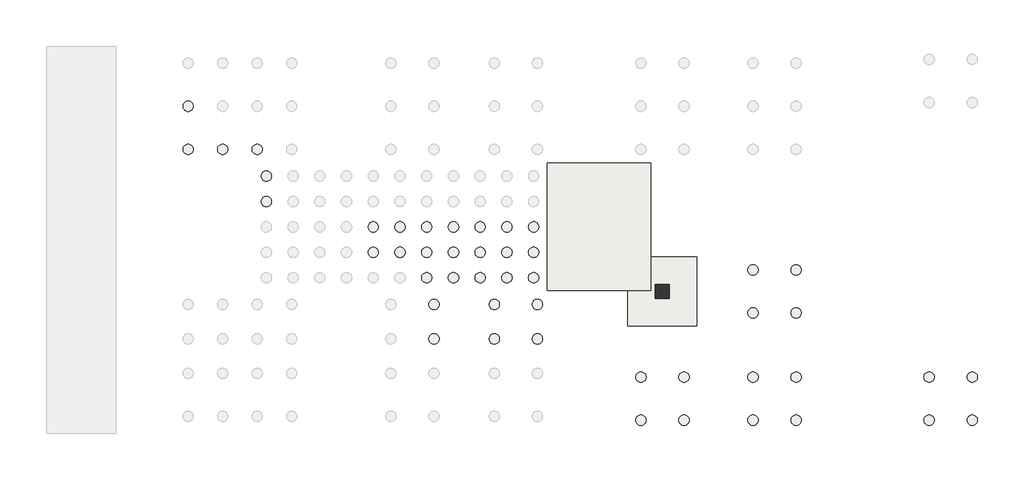
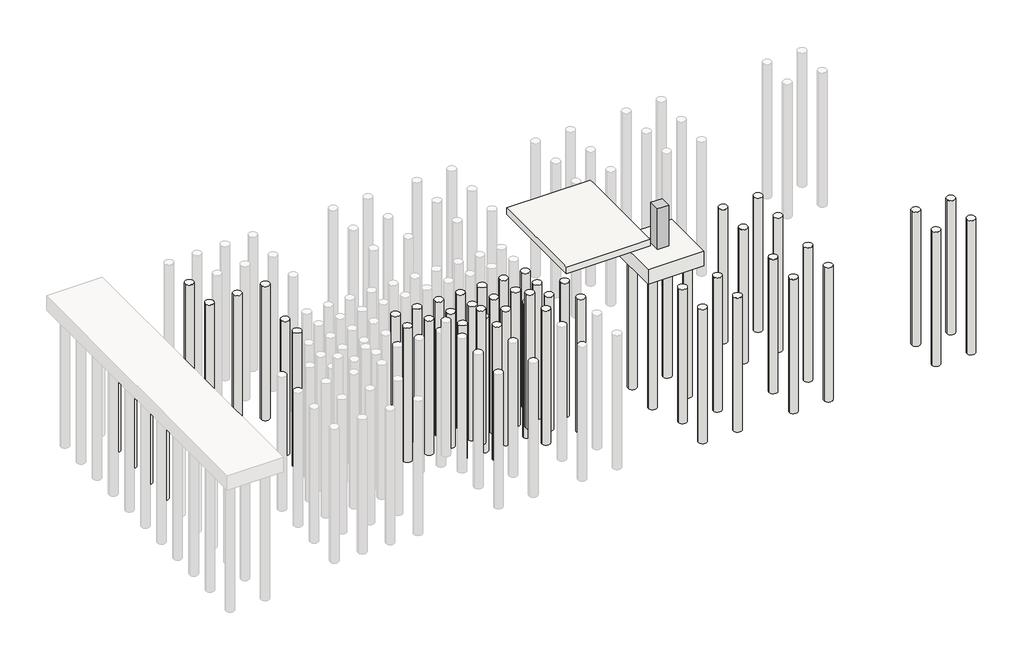
# One storey, part 2 of 3: 57 slabs, 1 column.
"""IFC4 building model written with IfcOpenShell, lengths in millimetres."""

from ifc_helpers import new_model, si_unit, point, frame, frame_2d, origin, place, context, project, spatial, polyline, circle_curve, trimmed, segment, composite_curve, outline, extrude, faceted_brep, element, save

model = new_model("IFC4")

# Units and contexts
model_context = context("Model", 3, world=origin())
ifc_project = project(units=[si_unit("LENGTHUNIT", "METRE", prefix="MILLI")], contexts=[model_context])

# Site, building, storey
site = spatial("IfcSite", under=ifc_project)
building = spatial("IfcBuilding", under=site)
storey = spatial("IfcBuildingStorey", under=building, Name="B.O.F(FDN)", Elevation=-2500.0279945)

# Column
placement = place(None, origin())
element("IfcColumn", 1, ObjectType="RC_Pedestal : H_SC_ACC_PED_W800xL800", at=placement, inside=storey, context=model_context, shape_type="SweptSolid", body=[
    extrude(outline(polyline([(33894.0, 26599.5208589), (33094.0, 26599.5208589), (33094.0, 27399.5208589), (33894.0, 27399.5208589), (33894.0, 26599.5208589)])), frame((0.0, 0.0, -2500.0279945), z_axis=(0.0, 0.0, 1.0), x_axis=(1.0, 0.0, 0.0)), (0.0, 0.0, 1.0), 3100.0),
])

# Slabs
element("IfcSlab", 2, ObjectType="H_SF_ACP_Pit Slab T500", at=placement, inside=storey, context=model_context, shape_type="Brep", body=[
    faceted_brep([(26830.0, 34449.5208589, -2400.0279945), (32830.0, 34449.5208589, -2400.0279945), (32830.0, 27049.5208589, -2400.0279945), (26830.0, 27049.5208589, -2400.0279945), (26830.0, 34449.5208589, -1900.0279945), (26830.0, 34059.5208589, -1900.0279945), (26830.0, 27439.5208589, -1900.0279945), (26830.0, 27049.5208589, -1900.0279945), (32830.0, 27049.5208589, -1900.0279945), (32830.0, 27439.5208589, -1900.0279945), (32830.0, 34059.5208589, -1900.0279945), (32830.0, 34449.5208589, -1900.0279945)], [[[0, 1, 2, 3]], [[4, 5, 6, 7, 8, 9, 10, 11]], [[1, 0, 4, 11]], [[2, 1, 11, 10, 9, 8]], [[3, 2, 8, 7]], [[0, 3, 7, 6, 5, 4]]]),
])
element("IfcSlab", 3, ObjectType="Foundation Rectangular(Non-Pile) : H_SF_ACF_W4000xL4000xT1100_Protection", at=placement, inside=storey, context=model_context, shape_type="SweptSolid", body=[
    extrude(outline(polyline([(35500.0, 28999.5208589), (35500.0, 24999.5208589), (31500.0, 24999.5208589), (31500.0, 28999.5208589), (35500.0, 28999.5208589)])), frame((0.0, 0.0, -3600.0279945), z_axis=(0.0, 0.0, 1.0), x_axis=(1.0, 0.0, 0.0)), (0.0, 0.0, 1.0), 1100.0),
])
element("IfcSlab", 4, ObjectType="Pile : H_SF_API_Steel Pile D508x12t_L10m", at=placement, inside=storey, context=model_context, shape_type="SweptSolid", body=[
    extrude(outline(composite_curve([segment(trimmed(circle_curve(frame_2d((1035.0, 38249.5208589)), 300.0), [point((1335.0, 38249.5208589))], [point((735.0, 38249.5208589))], False, "CARTESIAN"), True, "CONTINUOUS"), segment(trimmed(circle_curve(frame_2d((1035.0, 38249.5208589)), 300.0), [point((735.0, 38249.5208589))], [point((1335.0, 38249.5208589))], False, "CARTESIAN"), True, "CONTINUOUS")], self_intersect=False)), frame((0.0, 0.0, -13500.0279945), z_axis=(0.0, 0.0, 1.0), x_axis=(1.0, 0.0, 0.0)), (0.0, 0.0, 1.0), 10150.0),
])
element("IfcSlab", 5, ObjectType="Pile : H_SF_API_Steel Pile D508x12t_L10m", at=placement, inside=storey, context=model_context, shape_type="SweptSolid", body=[
    extrude(outline(composite_curve([segment(trimmed(circle_curve(frame_2d((1035.0, 36249.5208589)), 300.0), [point((1335.0, 36249.5208589))], [point((735.0, 36249.5208589))], False, "CARTESIAN"), True, "CONTINUOUS"), segment(trimmed(circle_curve(frame_2d((1035.0, 36249.5208589)), 300.0), [point((735.0, 36249.5208589))], [point((1335.0, 36249.5208589))], False, "CARTESIAN"), True, "CONTINUOUS")], self_intersect=False)), frame((0.0, 0.0, -13500.0279945), z_axis=(0.0, 0.0, 1.0), x_axis=(1.0, 0.0, 0.0)), (0.0, 0.0, 1.0), 10150.0),
])
element("IfcSlab", 6, ObjectType="Pile : H_SF_API_Steel Pile D508x12t_L10m", at=placement, inside=storey, context=model_context, shape_type="SweptSolid", body=[
    extrude(outline(composite_curve([segment(trimmed(circle_curve(frame_2d((1035.0, 34249.5208589)), 300.0), [point((1335.0, 34249.5208589))], [point((735.0, 34249.5208589))], False, "CARTESIAN"), True, "CONTINUOUS"), segment(trimmed(circle_curve(frame_2d((1035.0, 34249.5208589)), 300.0), [point((735.0, 34249.5208589))], [point((1335.0, 34249.5208589))], False, "CARTESIAN"), True, "CONTINUOUS")], self_intersect=False)), frame((0.0, 0.0, -13500.0279945), z_axis=(0.0, 0.0, 1.0), x_axis=(1.0, 0.0, 0.0)), (0.0, 0.0, 1.0), 10150.0),
])
element("IfcSlab", 7, ObjectType="Pile : H_SF_API_Steel Pile D508x12t_L10m", at=placement, inside=storey, context=model_context, shape_type="SweptSolid", body=[
    extrude(outline(composite_curve([segment(trimmed(circle_curve(frame_2d((1035.0, 32249.5208589)), 300.0), [point((1335.0, 32249.5208589))], [point((735.0, 32249.5208589))], False, "CARTESIAN"), True, "CONTINUOUS"), segment(trimmed(circle_curve(frame_2d((1035.0, 32249.5208589)), 300.0), [point((735.0, 32249.5208589))], [point((1335.0, 32249.5208589))], False, "CARTESIAN"), True, "CONTINUOUS")], self_intersect=False)), frame((0.0, 0.0, -13500.0279945), z_axis=(0.0, 0.0, 1.0), x_axis=(1.0, 0.0, 0.0)), (0.0, 0.0, 1.0), 10150.0),
])
element("IfcSlab", 8, ObjectType="Pile : H_SF_API_Steel Pile D508x12t_L10m", at=placement, inside=storey, context=model_context, shape_type="SweptSolid", body=[
    extrude(outline(composite_curve([segment(trimmed(circle_curve(frame_2d((20250.0, 24249.5208589)), 300.0), [point((20550.0, 24249.5208589))], [point((19950.0, 24249.5208589))], False, "CARTESIAN"), True, "CONTINUOUS"), segment(trimmed(circle_curve(frame_2d((20250.0, 24249.5208589)), 300.0), [point((19950.0, 24249.5208589))], [point((20550.0, 24249.5208589))], False, "CARTESIAN"), True, "CONTINUOUS")], self_intersect=False)), frame((0.0, 0.0, -12400.0279945), z_axis=(0.0, 0.0, 1.0), x_axis=(1.0, 0.0, 0.0)), (0.0, 0.0, 1.0), 10150.0),
])
element("IfcSlab", 9, ObjectType="Pile : H_SF_API_Steel Pile D508x12t_L10m", at=placement, inside=storey, context=model_context, shape_type="SweptSolid", body=[
    extrude(outline(composite_curve([segment(trimmed(circle_curve(frame_2d((20250.0, 26249.5208589)), 300.0), [point((20550.0, 26249.5208589))], [point((19950.0, 26249.5208589))], False, "CARTESIAN"), True, "CONTINUOUS"), segment(trimmed(circle_curve(frame_2d((20250.0, 26249.5208589)), 300.0), [point((19950.0, 26249.5208589))], [point((20550.0, 26249.5208589))], False, "CARTESIAN"), True, "CONTINUOUS")], self_intersect=False)), frame((0.0, 0.0, -12400.0279945), z_axis=(0.0, 0.0, 1.0), x_axis=(1.0, 0.0, 0.0)), (0.0, 0.0, 1.0), 10150.0),
])
element("IfcSlab", 10, ObjectType="Pile : H_SF_API_Steel Pile D508x12t_L10m", at=placement, inside=storey, context=model_context, shape_type="SweptSolid", body=[
    extrude(outline(composite_curve([segment(trimmed(circle_curve(frame_2d((23750.0, 24249.5208589)), 300.0), [point((23450.0, 24249.5208589))], [point((24050.0, 24249.5208589))], False, "CARTESIAN"), True, "CONTINUOUS"), segment(trimmed(circle_curve(frame_2d((23750.0, 24249.5208589)), 300.0), [point((24050.0, 24249.5208589))], [point((23450.0, 24249.5208589))], False, "CARTESIAN"), True, "CONTINUOUS")], self_intersect=False)), frame((0.0, 0.0, -12400.0279945), z_axis=(0.0, 0.0, 1.0), x_axis=(1.0, 0.0, 0.0)), (0.0, 0.0, 1.0), 10150.0),
])
element("IfcSlab", 11, ObjectType="Pile : H_SF_API_Steel Pile D508x12t_L10m", at=placement, inside=storey, context=model_context, shape_type="SweptSolid", body=[
    extrude(outline(composite_curve([segment(trimmed(circle_curve(frame_2d((26250.0, 26249.5208589)), 300.0), [point((26550.0, 26249.5208589))], [point((25950.0, 26249.5208589))], False, "CARTESIAN"), True, "CONTINUOUS"), segment(trimmed(circle_curve(frame_2d((26250.0, 26249.5208589)), 300.0), [point((25950.0, 26249.5208589))], [point((26550.0, 26249.5208589))], False, "CARTESIAN"), True, "CONTINUOUS")], self_intersect=False)), frame((0.0, 0.0, -12400.0279945), z_axis=(0.0, 0.0, 1.0), x_axis=(1.0, 0.0, 0.0)), (0.0, 0.0, 1.0), 10150.0),
])
element("IfcSlab", 12, ObjectType="Pile : H_SF_API_Steel Pile D508x12t_L10m", at=placement, inside=storey, context=model_context, shape_type="SweptSolid", body=[
    extrude(outline(composite_curve([segment(trimmed(circle_curve(frame_2d((23750.0, 26249.5208589)), 300.0), [point((23450.0, 26249.5208589))], [point((24050.0, 26249.5208589))], False, "CARTESIAN"), True, "CONTINUOUS"), segment(trimmed(circle_curve(frame_2d((23750.0, 26249.5208589)), 300.0), [point((24050.0, 26249.5208589))], [point((23450.0, 26249.5208589))], False, "CARTESIAN"), True, "CONTINUOUS")], self_intersect=False)), frame((0.0, 0.0, -12400.0279945), z_axis=(0.0, 0.0, 1.0), x_axis=(1.0, 0.0, 0.0)), (0.0, 0.0, 1.0), 10150.0),
])
element("IfcSlab", 13, ObjectType="Pile : H_SF_API_Steel Pile D508x12t_L10m", at=placement, inside=storey, context=model_context, shape_type="SweptSolid", body=[
    extrude(outline(composite_curve([segment(trimmed(circle_curve(frame_2d((34750.0, 19529.5208589)), 300.0), [point((35050.0, 19529.5208589))], [point((34450.0, 19529.5208589))], False, "CARTESIAN"), True, "CONTINUOUS"), segment(trimmed(circle_curve(frame_2d((34750.0, 19529.5208589)), 300.0), [point((34450.0, 19529.5208589))], [point((35050.0, 19529.5208589))], False, "CARTESIAN"), True, "CONTINUOUS")], self_intersect=False)), frame((0.0, 0.0, -12400.0279945), z_axis=(0.0, 0.0, 1.0), x_axis=(1.0, 0.0, 0.0)), (0.0, 0.0, 1.0), 10150.0),
])
element("IfcSlab", 14, ObjectType="Pile : H_SF_API_Steel Pile D508x12t_L10m", at=placement, inside=storey, context=model_context, shape_type="SweptSolid", body=[
    extrude(outline(composite_curve([segment(trimmed(circle_curve(frame_2d((32250.0, 19529.5208589)), 300.0), [point((31950.0, 19529.5208589))], [point((32550.0, 19529.5208589))], False, "CARTESIAN"), True, "CONTINUOUS"), segment(trimmed(circle_curve(frame_2d((32250.0, 19529.5208589)), 300.0), [point((32550.0, 19529.5208589))], [point((31950.0, 19529.5208589))], False, "CARTESIAN"), True, "CONTINUOUS")], self_intersect=False)), frame((0.0, 0.0, -12400.0279945), z_axis=(0.0, 0.0, 1.0), x_axis=(1.0, 0.0, 0.0)), (0.0, 0.0, 1.0), 10150.0),
])
element("IfcSlab", 15, ObjectType="Pile : H_SF_API_Steel Pile D508x12t_L10m", at=placement, inside=storey, context=model_context, shape_type="SweptSolid", body=[
    extrude(outline(composite_curve([segment(trimmed(circle_curve(frame_2d((34750.0, 22029.5208589)), 300.0), [point((35050.0, 22029.5208589))], [point((34450.0, 22029.5208589))], False, "CARTESIAN"), True, "CONTINUOUS"), segment(trimmed(circle_curve(frame_2d((34750.0, 22029.5208589)), 300.0), [point((34450.0, 22029.5208589))], [point((35050.0, 22029.5208589))], False, "CARTESIAN"), True, "CONTINUOUS")], self_intersect=False)), frame((0.0, 0.0, -12400.0279945), z_axis=(0.0, 0.0, 1.0), x_axis=(1.0, 0.0, 0.0)), (0.0, 0.0, 1.0), 10150.0),
])
element("IfcSlab", 16, ObjectType="Pile : H_SF_API_Steel Pile D508x12t_L10m", at=placement, inside=storey, context=model_context, shape_type="SweptSolid", body=[
    extrude(outline(composite_curve([segment(trimmed(circle_curve(frame_2d((32250.0, 22029.5208589)), 300.0), [point((31950.0, 22029.5208589))], [point((32550.0, 22029.5208589))], False, "CARTESIAN"), True, "CONTINUOUS"), segment(trimmed(circle_curve(frame_2d((32250.0, 22029.5208589)), 300.0), [point((32550.0, 22029.5208589))], [point((31950.0, 22029.5208589))], False, "CARTESIAN"), True, "CONTINUOUS")], self_intersect=False)), frame((0.0, 0.0, -12400.0279945), z_axis=(0.0, 0.0, 1.0), x_axis=(1.0, 0.0, 0.0)), (0.0, 0.0, 1.0), 10150.0),
])
element("IfcSlab", 17, ObjectType="Pile : H_SF_API_Steel Pile D508x12t_L10m", at=placement, inside=storey, context=model_context, shape_type="SweptSolid", body=[
    extrude(outline(composite_curve([segment(trimmed(circle_curve(frame_2d((34750.0, 25749.5208589)), 300.0), [point((35050.0, 25749.5208589))], [point((34450.0, 25749.5208589))], False, "CARTESIAN"), True, "CONTINUOUS"), segment(trimmed(circle_curve(frame_2d((34750.0, 25749.5208589)), 300.0), [point((34450.0, 25749.5208589))], [point((35050.0, 25749.5208589))], False, "CARTESIAN"), True, "CONTINUOUS")], self_intersect=False)), frame((0.0, 0.0, -13600.0279945), z_axis=(0.0, 0.0, 1.0), x_axis=(1.0, 0.0, 0.0)), (0.0, 0.0, 1.0), 10150.0),
])
element("IfcSlab", 18, ObjectType="Pile : H_SF_API_Steel Pile D508x12t_L10m", at=placement, inside=storey, context=model_context, shape_type="SweptSolid", body=[
    extrude(outline(composite_curve([segment(trimmed(circle_curve(frame_2d((32250.0, 25749.5208589)), 300.0), [point((31950.0, 25749.5208589))], [point((32550.0, 25749.5208589))], False, "CARTESIAN"), True, "CONTINUOUS"), segment(trimmed(circle_curve(frame_2d((32250.0, 25749.5208589)), 300.0), [point((32550.0, 25749.5208589))], [point((31950.0, 25749.5208589))], False, "CARTESIAN"), True, "CONTINUOUS")], self_intersect=False)), frame((0.0, 0.0, -13600.0279945), z_axis=(0.0, 0.0, 1.0), x_axis=(1.0, 0.0, 0.0)), (0.0, 0.0, 1.0), 10150.0),
])
element("IfcSlab", 19, ObjectType="Pile : H_SF_API_Steel Pile D508x12t_L10m", at=placement, inside=storey, context=model_context, shape_type="SweptSolid", body=[
    extrude(outline(composite_curve([segment(trimmed(circle_curve(frame_2d((34750.0, 28249.5208589)), 300.0), [point((35050.0, 28249.5208589))], [point((34450.0, 28249.5208589))], False, "CARTESIAN"), True, "CONTINUOUS"), segment(trimmed(circle_curve(frame_2d((34750.0, 28249.5208589)), 300.0), [point((34450.0, 28249.5208589))], [point((35050.0, 28249.5208589))], False, "CARTESIAN"), True, "CONTINUOUS")], self_intersect=False)), frame((0.0, 0.0, -13600.0279945), z_axis=(0.0, 0.0, 1.0), x_axis=(1.0, 0.0, 0.0)), (0.0, 0.0, 1.0), 10150.0),
])
element("IfcSlab", 20, ObjectType="Pile : H_SF_API_Steel Pile D508x12t_L10m", at=placement, inside=storey, context=model_context, shape_type="SweptSolid", body=[
    extrude(outline(composite_curve([segment(trimmed(circle_curve(frame_2d((32250.0, 28249.5208589)), 300.0), [point((31950.0, 28249.5208589))], [point((32550.0, 28249.5208589))], False, "CARTESIAN"), True, "CONTINUOUS"), segment(trimmed(circle_curve(frame_2d((32250.0, 28249.5208589)), 300.0), [point((32550.0, 28249.5208589))], [point((31950.0, 28249.5208589))], False, "CARTESIAN"), True, "CONTINUOUS")], self_intersect=False)), frame((0.0, 0.0, -13600.0279945), z_axis=(0.0, 0.0, 1.0), x_axis=(1.0, 0.0, 0.0)), (0.0, 0.0, 1.0), 10150.0),
])
element("IfcSlab", 21, ObjectType="Pile : H_SF_API_Steel Pile D508x12t_L10m", at=placement, inside=storey, context=model_context, shape_type="SweptSolid", body=[
    extrude(outline(composite_curve([segment(trimmed(circle_curve(frame_2d((41250.0, 25749.5208589)), 300.0), [point((41550.0, 25749.5208589))], [point((40950.0, 25749.5208589))], False, "CARTESIAN"), True, "CONTINUOUS"), segment(trimmed(circle_curve(frame_2d((41250.0, 25749.5208589)), 300.0), [point((40950.0, 25749.5208589))], [point((41550.0, 25749.5208589))], False, "CARTESIAN"), True, "CONTINUOUS")], self_intersect=False)), frame((0.0, 0.0, -12400.0279945), z_axis=(0.0, 0.0, 1.0), x_axis=(1.0, 0.0, 0.0)), (0.0, 0.0, 1.0), 10150.0),
])
element("IfcSlab", 22, ObjectType="Pile : H_SF_API_Steel Pile D508x12t_L10m", at=placement, inside=storey, context=model_context, shape_type="SweptSolid", body=[
    extrude(outline(composite_curve([segment(trimmed(circle_curve(frame_2d((38750.0, 25749.5208589)), 300.0), [point((38450.0, 25749.5208589))], [point((39050.0, 25749.5208589))], False, "CARTESIAN"), True, "CONTINUOUS"), segment(trimmed(circle_curve(frame_2d((38750.0, 25749.5208589)), 300.0), [point((39050.0, 25749.5208589))], [point((38450.0, 25749.5208589))], False, "CARTESIAN"), True, "CONTINUOUS")], self_intersect=False)), frame((0.0, 0.0, -12400.0279945), z_axis=(0.0, 0.0, 1.0), x_axis=(1.0, 0.0, 0.0)), (0.0, 0.0, 1.0), 10150.0),
])
element("IfcSlab", 23, ObjectType="Pile : H_SF_API_Steel Pile D508x12t_L10m", at=placement, inside=storey, context=model_context, shape_type="SweptSolid", body=[
    extrude(outline(composite_curve([segment(trimmed(circle_curve(frame_2d((41250.0, 28249.5208589)), 300.0), [point((41550.0, 28249.5208589))], [point((40950.0, 28249.5208589))], False, "CARTESIAN"), True, "CONTINUOUS"), segment(trimmed(circle_curve(frame_2d((41250.0, 28249.5208589)), 300.0), [point((40950.0, 28249.5208589))], [point((41550.0, 28249.5208589))], False, "CARTESIAN"), True, "CONTINUOUS")], self_intersect=False)), frame((0.0, 0.0, -12400.0279945), z_axis=(0.0, 0.0, 1.0), x_axis=(1.0, 0.0, 0.0)), (0.0, 0.0, 1.0), 10150.0),
])
element("IfcSlab", 24, ObjectType="Pile : H_SF_API_Steel Pile D508x12t_L10m", at=placement, inside=storey, context=model_context, shape_type="SweptSolid", body=[
    extrude(outline(composite_curve([segment(trimmed(circle_curve(frame_2d((38750.0, 28249.5208589)), 300.0), [point((38450.0, 28249.5208589))], [point((39050.0, 28249.5208589))], False, "CARTESIAN"), True, "CONTINUOUS"), segment(trimmed(circle_curve(frame_2d((38750.0, 28249.5208589)), 300.0), [point((39050.0, 28249.5208589))], [point((38450.0, 28249.5208589))], False, "CARTESIAN"), True, "CONTINUOUS")], self_intersect=False)), frame((0.0, 0.0, -12400.0279945), z_axis=(0.0, 0.0, 1.0), x_axis=(1.0, 0.0, 0.0)), (0.0, 0.0, 1.0), 10150.0),
])
element("IfcSlab", 25, ObjectType="Pile : H_SF_API_Steel Pile D508x12t_L10m", at=placement, inside=storey, context=model_context, shape_type="SweptSolid", body=[
    extrude(outline(composite_curve([segment(trimmed(circle_curve(frame_2d((41250.0, 19529.5208589)), 300.0), [point((41550.0, 19529.5208589))], [point((40950.0, 19529.5208589))], False, "CARTESIAN"), True, "CONTINUOUS"), segment(trimmed(circle_curve(frame_2d((41250.0, 19529.5208589)), 300.0), [point((40950.0, 19529.5208589))], [point((41550.0, 19529.5208589))], False, "CARTESIAN"), True, "CONTINUOUS")], self_intersect=False)), frame((0.0, 0.0, -12400.0279945), z_axis=(0.0, 0.0, 1.0), x_axis=(1.0, 0.0, 0.0)), (0.0, 0.0, 1.0), 10150.0),
])
element("IfcSlab", 26, ObjectType="Pile : H_SF_API_Steel Pile D508x12t_L10m", at=placement, inside=storey, context=model_context, shape_type="SweptSolid", body=[
    extrude(outline(composite_curve([segment(trimmed(circle_curve(frame_2d((38750.0, 19529.5208589)), 300.0), [point((38450.0, 19529.5208589))], [point((39050.0, 19529.5208589))], False, "CARTESIAN"), True, "CONTINUOUS"), segment(trimmed(circle_curve(frame_2d((38750.0, 19529.5208589)), 300.0), [point((39050.0, 19529.5208589))], [point((38450.0, 19529.5208589))], False, "CARTESIAN"), True, "CONTINUOUS")], self_intersect=False)), frame((0.0, 0.0, -12400.0279945), z_axis=(0.0, 0.0, 1.0), x_axis=(1.0, 0.0, 0.0)), (0.0, 0.0, 1.0), 10150.0),
])
element("IfcSlab", 27, ObjectType="Pile : H_SF_API_Steel Pile D508x12t_L10m", at=placement, inside=storey, context=model_context, shape_type="SweptSolid", body=[
    extrude(outline(composite_curve([segment(trimmed(circle_curve(frame_2d((41250.0, 22029.5208589)), 300.0), [point((41550.0, 22029.5208589))], [point((40950.0, 22029.5208589))], False, "CARTESIAN"), True, "CONTINUOUS"), segment(trimmed(circle_curve(frame_2d((41250.0, 22029.5208589)), 300.0), [point((40950.0, 22029.5208589))], [point((41550.0, 22029.5208589))], False, "CARTESIAN"), True, "CONTINUOUS")], self_intersect=False)), frame((0.0, 0.0, -12400.0279945), z_axis=(0.0, 0.0, 1.0), x_axis=(1.0, 0.0, 0.0)), (0.0, 0.0, 1.0), 10150.0),
])
element("IfcSlab", 28, ObjectType="Pile : H_SF_API_Steel Pile D508x12t_L10m", at=placement, inside=storey, context=model_context, shape_type="SweptSolid", body=[
    extrude(outline(composite_curve([segment(trimmed(circle_curve(frame_2d((38750.0, 22029.5208589)), 300.0), [point((38450.0, 22029.5208589))], [point((39050.0, 22029.5208589))], False, "CARTESIAN"), True, "CONTINUOUS"), segment(trimmed(circle_curve(frame_2d((38750.0, 22029.5208589)), 300.0), [point((39050.0, 22029.5208589))], [point((38450.0, 22029.5208589))], False, "CARTESIAN"), True, "CONTINUOUS")], self_intersect=False)), frame((0.0, 0.0, -12400.0279945), z_axis=(0.0, 0.0, 1.0), x_axis=(1.0, 0.0, 0.0)), (0.0, 0.0, 1.0), 10150.0),
])
element("IfcSlab", 29, ObjectType="Pile : H_SF_API_Steel Pile D508x12t_L10m", at=placement, inside=storey, context=model_context, shape_type="SweptSolid", body=[
    extrude(outline(composite_curve([segment(trimmed(circle_curve(frame_2d((51465.0, 19529.5208589)), 300.0), [point((51765.0, 19529.5208589))], [point((51165.0, 19529.5208589))], False, "CARTESIAN"), True, "CONTINUOUS"), segment(trimmed(circle_curve(frame_2d((51465.0, 19529.5208589)), 300.0), [point((51165.0, 19529.5208589))], [point((51765.0, 19529.5208589))], False, "CARTESIAN"), True, "CONTINUOUS")], self_intersect=False)), frame((0.0, 0.0, -12400.0279945), z_axis=(0.0, 0.0, 1.0), x_axis=(1.0, 0.0, 0.0)), (0.0, 0.0, 1.0), 10150.0),
])
element("IfcSlab", 30, ObjectType="Pile : H_SF_API_Steel Pile D508x12t_L10m", at=placement, inside=storey, context=model_context, shape_type="SweptSolid", body=[
    extrude(outline(composite_curve([segment(trimmed(circle_curve(frame_2d((48965.0, 19529.5208589)), 300.0), [point((48665.0, 19529.5208589))], [point((49265.0, 19529.5208589))], False, "CARTESIAN"), True, "CONTINUOUS"), segment(trimmed(circle_curve(frame_2d((48965.0, 19529.5208589)), 300.0), [point((49265.0, 19529.5208589))], [point((48665.0, 19529.5208589))], False, "CARTESIAN"), True, "CONTINUOUS")], self_intersect=False)), frame((0.0, 0.0, -12400.0279945), z_axis=(0.0, 0.0, 1.0), x_axis=(1.0, 0.0, 0.0)), (0.0, 0.0, 1.0), 10150.0),
])
element("IfcSlab", 31, ObjectType="Pile : H_SF_API_Steel Pile D508x12t_L10m", at=placement, inside=storey, context=model_context, shape_type="SweptSolid", body=[
    extrude(outline(composite_curve([segment(trimmed(circle_curve(frame_2d((51465.0, 22029.5208589)), 300.0), [point((51765.0, 22029.5208589))], [point((51165.0, 22029.5208589))], False, "CARTESIAN"), True, "CONTINUOUS"), segment(trimmed(circle_curve(frame_2d((51465.0, 22029.5208589)), 300.0), [point((51165.0, 22029.5208589))], [point((51765.0, 22029.5208589))], False, "CARTESIAN"), True, "CONTINUOUS")], self_intersect=False)), frame((0.0, 0.0, -12400.0279945), z_axis=(0.0, 0.0, 1.0), x_axis=(1.0, 0.0, 0.0)), (0.0, 0.0, 1.0), 10150.0),
])
element("IfcSlab", 32, ObjectType="Pile : H_SF_API_Steel Pile D508x12t_L10m", at=placement, inside=storey, context=model_context, shape_type="SweptSolid", body=[
    extrude(outline(composite_curve([segment(trimmed(circle_curve(frame_2d((48965.0, 22029.5208589)), 300.0), [point((48665.0, 22029.5208589))], [point((49265.0, 22029.5208589))], False, "CARTESIAN"), True, "CONTINUOUS"), segment(trimmed(circle_curve(frame_2d((48965.0, 22029.5208589)), 300.0), [point((49265.0, 22029.5208589))], [point((48665.0, 22029.5208589))], False, "CARTESIAN"), True, "CONTINUOUS")], self_intersect=False)), frame((0.0, 0.0, -12400.0279945), z_axis=(0.0, 0.0, 1.0), x_axis=(1.0, 0.0, 0.0)), (0.0, 0.0, 1.0), 10150.0),
])
element("IfcSlab", 33, ObjectType="Pile : H_SF_API_Steel Pile D508x12t_L10m", at=placement, inside=storey, context=model_context, shape_type="SweptSolid", body=[
    extrude(outline(composite_curve([segment(trimmed(circle_curve(frame_2d((6000.0, 37749.5208589)), 300.0), [point((5700.0, 37749.5208589))], [point((6300.0, 37749.5208589))], False, "CARTESIAN"), True, "CONTINUOUS"), segment(trimmed(circle_curve(frame_2d((6000.0, 37749.5208589)), 300.0), [point((6300.0, 37749.5208589))], [point((5700.0, 37749.5208589))], False, "CARTESIAN"), True, "CONTINUOUS")], self_intersect=False)), frame((0.0, 0.0, -12400.0279945), z_axis=(0.0, 0.0, 1.0), x_axis=(1.0, 0.0, 0.0)), (0.0, 0.0, 1.0), 10150.0),
])
element("IfcSlab", 34, ObjectType="Pile : H_SF_API_Steel Pile D508x12t_L10m", at=placement, inside=storey, context=model_context, shape_type="SweptSolid", body=[
    extrude(outline(composite_curve([segment(trimmed(circle_curve(frame_2d((6000.0, 35249.5208589)), 300.0), [point((5700.0, 35249.5208589))], [point((6300.0, 35249.5208589))], False, "CARTESIAN"), True, "CONTINUOUS"), segment(trimmed(circle_curve(frame_2d((6000.0, 35249.5208589)), 300.0), [point((6300.0, 35249.5208589))], [point((5700.0, 35249.5208589))], False, "CARTESIAN"), True, "CONTINUOUS")], self_intersect=False)), frame((0.0, 0.0, -12400.0279945), z_axis=(0.0, 0.0, 1.0), x_axis=(1.0, 0.0, 0.0)), (0.0, 0.0, 1.0), 10150.0),
])
element("IfcSlab", 35, ObjectType="Pile : H_SF_API_Steel Pile D508x12t_L10m", at=placement, inside=storey, context=model_context, shape_type="SweptSolid", body=[
    extrude(outline(composite_curve([segment(trimmed(circle_curve(frame_2d((8000.0, 35249.5208589)), 300.0), [point((8300.0, 35249.5208589))], [point((7700.0, 35249.5208589))], False, "CARTESIAN"), True, "CONTINUOUS"), segment(trimmed(circle_curve(frame_2d((8000.0, 35249.5208589)), 300.0), [point((7700.0, 35249.5208589))], [point((8300.0, 35249.5208589))], False, "CARTESIAN"), True, "CONTINUOUS")], self_intersect=False)), frame((0.0, 0.0, -12400.0279945), z_axis=(0.0, 0.0, 1.0), x_axis=(1.0, 0.0, 0.0)), (0.0, 0.0, 1.0), 10150.0),
])
element("IfcSlab", 36, ObjectType="Pile : H_SF_API_Steel Pile D508x12t_L10m", at=placement, inside=storey, context=model_context, shape_type="SweptSolid", body=[
    extrude(outline(composite_curve([segment(trimmed(circle_curve(frame_2d((10000.0, 35249.5208589)), 300.0), [point((9700.0, 35249.5208589))], [point((10300.0, 35249.5208589))], False, "CARTESIAN"), True, "CONTINUOUS"), segment(trimmed(circle_curve(frame_2d((10000.0, 35249.5208589)), 300.0), [point((10300.0, 35249.5208589))], [point((9700.0, 35249.5208589))], False, "CARTESIAN"), True, "CONTINUOUS")], self_intersect=False)), frame((0.0, 0.0, -12400.0279945), z_axis=(0.0, 0.0, 1.0), x_axis=(1.0, 0.0, 0.0)), (0.0, 0.0, 1.0), 10150.0),
])
element("IfcSlab", 37, ObjectType="Pile : H_SF_API_Steel Pile D508x12t_L10m", at=placement, inside=storey, context=model_context, shape_type="SweptSolid", body=[
    extrude(outline(composite_curve([segment(trimmed(circle_curve(frame_2d((10530.0, 33699.5208589)), 300.0), [point((10230.0, 33699.5208589))], [point((10830.0, 33699.5208589))], False, "CARTESIAN"), True, "CONTINUOUS"), segment(trimmed(circle_curve(frame_2d((10530.0, 33699.5208589)), 300.0), [point((10830.0, 33699.5208589))], [point((10230.0, 33699.5208589))], False, "CARTESIAN"), True, "CONTINUOUS")], self_intersect=False)), frame((0.0, 0.0, -14300.0279945), z_axis=(0.0, 0.0, 1.0), x_axis=(1.0, 0.0, 0.0)), (0.0, 0.0, 1.0), 10150.0),
])
element("IfcSlab", 38, ObjectType="Pile : H_SF_API_Steel Pile D508x12t_L10m", at=placement, inside=storey, context=model_context, shape_type="SweptSolid", body=[
    extrude(outline(composite_curve([segment(trimmed(circle_curve(frame_2d((10530.0, 32224.5208589)), 300.0), [point((10230.0, 32224.5208589))], [point((10830.0, 32224.5208589))], False, "CARTESIAN"), True, "CONTINUOUS"), segment(trimmed(circle_curve(frame_2d((10530.0, 32224.5208589)), 300.0), [point((10830.0, 32224.5208589))], [point((10230.0, 32224.5208589))], False, "CARTESIAN"), True, "CONTINUOUS")], self_intersect=False)), frame((0.0, 0.0, -14300.0279945), z_axis=(0.0, 0.0, 1.0), x_axis=(1.0, 0.0, 0.0)), (0.0, 0.0, 1.0), 10150.0),
])
element("IfcSlab", 39, ObjectType="Pile : H_SF_API_Steel Pile D508x12t_L10m", at=placement, inside=storey, context=model_context, shape_type="SweptSolid", body=[
    extrude(outline(composite_curve([segment(trimmed(circle_curve(frame_2d((26030.0, 27799.5208589)), 300.0), [point((26330.0, 27799.5208589))], [point((25730.0, 27799.5208589))], False, "CARTESIAN"), True, "CONTINUOUS"), segment(trimmed(circle_curve(frame_2d((26030.0, 27799.5208589)), 300.0), [point((25730.0, 27799.5208589))], [point((26330.0, 27799.5208589))], False, "CARTESIAN"), True, "CONTINUOUS")], self_intersect=False)), frame((0.0, 0.0, -14300.0279945), z_axis=(0.0, 0.0, 1.0), x_axis=(1.0, 0.0, 0.0)), (0.0, 0.0, 1.0), 10150.0),
])
element("IfcSlab", 40, ObjectType="Pile : H_SF_API_Steel Pile D508x12t_L10m", at=placement, inside=storey, context=model_context, shape_type="SweptSolid", body=[
    extrude(outline(composite_curve([segment(trimmed(circle_curve(frame_2d((26030.0, 29274.5208589)), 300.0), [point((26330.0, 29274.5208589))], [point((25730.0, 29274.5208589))], False, "CARTESIAN"), True, "CONTINUOUS"), segment(trimmed(circle_curve(frame_2d((26030.0, 29274.5208589)), 300.0), [point((25730.0, 29274.5208589))], [point((26330.0, 29274.5208589))], False, "CARTESIAN"), True, "CONTINUOUS")], self_intersect=False)), frame((0.0, 0.0, -14300.0279945), z_axis=(0.0, 0.0, 1.0), x_axis=(1.0, 0.0, 0.0)), (0.0, 0.0, 1.0), 10150.0),
])
element("IfcSlab", 41, ObjectType="Pile : H_SF_API_Steel Pile D508x12t_L10m", at=placement, inside=storey, context=model_context, shape_type="SweptSolid", body=[
    extrude(outline(composite_curve([segment(trimmed(circle_curve(frame_2d((26030.0, 30749.5208589)), 300.0), [point((26330.0, 30749.5208589))], [point((25730.0, 30749.5208589))], False, "CARTESIAN"), True, "CONTINUOUS"), segment(trimmed(circle_curve(frame_2d((26030.0, 30749.5208589)), 300.0), [point((25730.0, 30749.5208589))], [point((26330.0, 30749.5208589))], False, "CARTESIAN"), True, "CONTINUOUS")], self_intersect=False)), frame((0.0, 0.0, -14300.0279945), z_axis=(0.0, 0.0, 1.0), x_axis=(1.0, 0.0, 0.0)), (0.0, 0.0, 1.0), 10150.0),
])
element("IfcSlab", 42, ObjectType="Pile : H_SF_API_Steel Pile D508x12t_L10m", at=placement, inside=storey, context=model_context, shape_type="SweptSolid", body=[
    extrude(outline(composite_curve([segment(trimmed(circle_curve(frame_2d((24480.0, 27799.5208589)), 300.0), [point((24780.0, 27799.5208589))], [point((24180.0, 27799.5208589))], False, "CARTESIAN"), True, "CONTINUOUS"), segment(trimmed(circle_curve(frame_2d((24480.0, 27799.5208589)), 300.0), [point((24180.0, 27799.5208589))], [point((24780.0, 27799.5208589))], False, "CARTESIAN"), True, "CONTINUOUS")], self_intersect=False)), frame((0.0, 0.0, -14300.0279945), z_axis=(0.0, 0.0, 1.0), x_axis=(1.0, 0.0, 0.0)), (0.0, 0.0, 1.0), 10150.0),
])
element("IfcSlab", 43, ObjectType="Pile : H_SF_API_Steel Pile D508x12t_L10m", at=placement, inside=storey, context=model_context, shape_type="SweptSolid", body=[
    extrude(outline(composite_curve([segment(trimmed(circle_curve(frame_2d((24480.0, 29274.5208589)), 300.0), [point((24780.0, 29274.5208589))], [point((24180.0, 29274.5208589))], False, "CARTESIAN"), True, "CONTINUOUS"), segment(trimmed(circle_curve(frame_2d((24480.0, 29274.5208589)), 300.0), [point((24180.0, 29274.5208589))], [point((24780.0, 29274.5208589))], False, "CARTESIAN"), True, "CONTINUOUS")], self_intersect=False)), frame((0.0, 0.0, -14300.0279945), z_axis=(0.0, 0.0, 1.0), x_axis=(1.0, 0.0, 0.0)), (0.0, 0.0, 1.0), 10150.0),
])
element("IfcSlab", 44, ObjectType="Pile : H_SF_API_Steel Pile D508x12t_L10m", at=placement, inside=storey, context=model_context, shape_type="SweptSolid", body=[
    extrude(outline(composite_curve([segment(trimmed(circle_curve(frame_2d((24480.0, 30749.5208589)), 300.0), [point((24780.0, 30749.5208589))], [point((24180.0, 30749.5208589))], False, "CARTESIAN"), True, "CONTINUOUS"), segment(trimmed(circle_curve(frame_2d((24480.0, 30749.5208589)), 300.0), [point((24180.0, 30749.5208589))], [point((24780.0, 30749.5208589))], False, "CARTESIAN"), True, "CONTINUOUS")], self_intersect=False)), frame((0.0, 0.0, -14300.0279945), z_axis=(0.0, 0.0, 1.0), x_axis=(1.0, 0.0, 0.0)), (0.0, 0.0, 1.0), 10150.0),
])
element("IfcSlab", 45, ObjectType="Pile : H_SF_API_Steel Pile D508x12t_L10m", at=placement, inside=storey, context=model_context, shape_type="SweptSolid", body=[
    extrude(outline(composite_curve([segment(trimmed(circle_curve(frame_2d((22930.0, 27799.5208589)), 300.0), [point((23230.0, 27799.5208589))], [point((22630.0, 27799.5208589))], False, "CARTESIAN"), True, "CONTINUOUS"), segment(trimmed(circle_curve(frame_2d((22930.0, 27799.5208589)), 300.0), [point((22630.0, 27799.5208589))], [point((23230.0, 27799.5208589))], False, "CARTESIAN"), True, "CONTINUOUS")], self_intersect=False)), frame((0.0, 0.0, -14300.0279945), z_axis=(0.0, 0.0, 1.0), x_axis=(1.0, 0.0, 0.0)), (0.0, 0.0, 1.0), 10150.0),
])
element("IfcSlab", 46, ObjectType="Pile : H_SF_API_Steel Pile D508x12t_L10m", at=placement, inside=storey, context=model_context, shape_type="SweptSolid", body=[
    extrude(outline(composite_curve([segment(trimmed(circle_curve(frame_2d((22930.0, 29274.5208589)), 300.0), [point((23230.0, 29274.5208589))], [point((22630.0, 29274.5208589))], False, "CARTESIAN"), True, "CONTINUOUS"), segment(trimmed(circle_curve(frame_2d((22930.0, 29274.5208589)), 300.0), [point((22630.0, 29274.5208589))], [point((23230.0, 29274.5208589))], False, "CARTESIAN"), True, "CONTINUOUS")], self_intersect=False)), frame((0.0, 0.0, -14300.0279945), z_axis=(0.0, 0.0, 1.0), x_axis=(1.0, 0.0, 0.0)), (0.0, 0.0, 1.0), 10150.0),
])
element("IfcSlab", 47, ObjectType="Pile : H_SF_API_Steel Pile D508x12t_L10m", at=placement, inside=storey, context=model_context, shape_type="SweptSolid", body=[
    extrude(outline(composite_curve([segment(trimmed(circle_curve(frame_2d((22930.0, 30749.5208589)), 300.0), [point((23230.0, 30749.5208589))], [point((22630.0, 30749.5208589))], False, "CARTESIAN"), True, "CONTINUOUS"), segment(trimmed(circle_curve(frame_2d((22930.0, 30749.5208589)), 300.0), [point((22630.0, 30749.5208589))], [point((23230.0, 30749.5208589))], False, "CARTESIAN"), True, "CONTINUOUS")], self_intersect=False)), frame((0.0, 0.0, -14300.0279945), z_axis=(0.0, 0.0, 1.0), x_axis=(1.0, 0.0, 0.0)), (0.0, 0.0, 1.0), 10150.0),
])
element("IfcSlab", 48, ObjectType="Pile : H_SF_API_Steel Pile D508x12t_L10m", at=placement, inside=storey, context=model_context, shape_type="SweptSolid", body=[
    extrude(outline(composite_curve([segment(trimmed(circle_curve(frame_2d((21380.0, 27799.5208589)), 300.0), [point((21680.0, 27799.5208589))], [point((21080.0, 27799.5208589))], False, "CARTESIAN"), True, "CONTINUOUS"), segment(trimmed(circle_curve(frame_2d((21380.0, 27799.5208589)), 300.0), [point((21080.0, 27799.5208589))], [point((21680.0, 27799.5208589))], False, "CARTESIAN"), True, "CONTINUOUS")], self_intersect=False)), frame((0.0, 0.0, -14300.0279945), z_axis=(0.0, 0.0, 1.0), x_axis=(1.0, 0.0, 0.0)), (0.0, 0.0, 1.0), 10150.0),
])
element("IfcSlab", 49, ObjectType="Pile : H_SF_API_Steel Pile D508x12t_L10m", at=placement, inside=storey, context=model_context, shape_type="SweptSolid", body=[
    extrude(outline(composite_curve([segment(trimmed(circle_curve(frame_2d((21380.0, 29274.5208589)), 300.0), [point((21680.0, 29274.5208589))], [point((21080.0, 29274.5208589))], False, "CARTESIAN"), True, "CONTINUOUS"), segment(trimmed(circle_curve(frame_2d((21380.0, 29274.5208589)), 300.0), [point((21080.0, 29274.5208589))], [point((21680.0, 29274.5208589))], False, "CARTESIAN"), True, "CONTINUOUS")], self_intersect=False)), frame((0.0, 0.0, -14300.0279945), z_axis=(0.0, 0.0, 1.0), x_axis=(1.0, 0.0, 0.0)), (0.0, 0.0, 1.0), 10150.0),
])
element("IfcSlab", 50, ObjectType="Pile : H_SF_API_Steel Pile D508x12t_L10m", at=placement, inside=storey, context=model_context, shape_type="SweptSolid", body=[
    extrude(outline(composite_curve([segment(trimmed(circle_curve(frame_2d((21380.0, 30749.5208589)), 300.0), [point((21680.0, 30749.5208589))], [point((21080.0, 30749.5208589))], False, "CARTESIAN"), True, "CONTINUOUS"), segment(trimmed(circle_curve(frame_2d((21380.0, 30749.5208589)), 300.0), [point((21080.0, 30749.5208589))], [point((21680.0, 30749.5208589))], False, "CARTESIAN"), True, "CONTINUOUS")], self_intersect=False)), frame((0.0, 0.0, -14300.0279945), z_axis=(0.0, 0.0, 1.0), x_axis=(1.0, 0.0, 0.0)), (0.0, 0.0, 1.0), 10150.0),
])
element("IfcSlab", 51, ObjectType="Pile : H_SF_API_Steel Pile D508x12t_L10m", at=placement, inside=storey, context=model_context, shape_type="SweptSolid", body=[
    extrude(outline(composite_curve([segment(trimmed(circle_curve(frame_2d((19830.0, 27799.5208589)), 300.0), [point((20130.0, 27799.5208589))], [point((19530.0, 27799.5208589))], False, "CARTESIAN"), True, "CONTINUOUS"), segment(trimmed(circle_curve(frame_2d((19830.0, 27799.5208589)), 300.0), [point((19530.0, 27799.5208589))], [point((20130.0, 27799.5208589))], False, "CARTESIAN"), True, "CONTINUOUS")], self_intersect=False)), frame((0.0, 0.0, -14300.0279945), z_axis=(0.0, 0.0, 1.0), x_axis=(1.0, 0.0, 0.0)), (0.0, 0.0, 1.0), 10150.0),
])
element("IfcSlab", 52, ObjectType="Pile : H_SF_API_Steel Pile D508x12t_L10m", at=placement, inside=storey, context=model_context, shape_type="SweptSolid", body=[
    extrude(outline(composite_curve([segment(trimmed(circle_curve(frame_2d((19830.0, 29274.5208589)), 300.0), [point((20130.0, 29274.5208589))], [point((19530.0, 29274.5208589))], False, "CARTESIAN"), True, "CONTINUOUS"), segment(trimmed(circle_curve(frame_2d((19830.0, 29274.5208589)), 300.0), [point((19530.0, 29274.5208589))], [point((20130.0, 29274.5208589))], False, "CARTESIAN"), True, "CONTINUOUS")], self_intersect=False)), frame((0.0, 0.0, -14300.0279945), z_axis=(0.0, 0.0, 1.0), x_axis=(1.0, 0.0, 0.0)), (0.0, 0.0, 1.0), 10150.0),
])
element("IfcSlab", 53, ObjectType="Pile : H_SF_API_Steel Pile D508x12t_L10m", at=placement, inside=storey, context=model_context, shape_type="SweptSolid", body=[
    extrude(outline(composite_curve([segment(trimmed(circle_curve(frame_2d((19830.0, 30749.5208589)), 300.0), [point((20130.0, 30749.5208589))], [point((19530.0, 30749.5208589))], False, "CARTESIAN"), True, "CONTINUOUS"), segment(trimmed(circle_curve(frame_2d((19830.0, 30749.5208589)), 300.0), [point((19530.0, 30749.5208589))], [point((20130.0, 30749.5208589))], False, "CARTESIAN"), True, "CONTINUOUS")], self_intersect=False)), frame((0.0, 0.0, -14300.0279945), z_axis=(0.0, 0.0, 1.0), x_axis=(1.0, 0.0, 0.0)), (0.0, 0.0, 1.0), 10150.0),
])
element("IfcSlab", 54, ObjectType="Pile : H_SF_API_Steel Pile D508x12t_L10m", at=placement, inside=storey, context=model_context, shape_type="SweptSolid", body=[
    extrude(outline(composite_curve([segment(trimmed(circle_curve(frame_2d((18280.0, 29274.5208589)), 300.0), [point((18580.0, 29274.5208589))], [point((17980.0, 29274.5208589))], False, "CARTESIAN"), True, "CONTINUOUS"), segment(trimmed(circle_curve(frame_2d((18280.0, 29274.5208589)), 300.0), [point((17980.0, 29274.5208589))], [point((18580.0, 29274.5208589))], False, "CARTESIAN"), True, "CONTINUOUS")], self_intersect=False)), frame((0.0, 0.0, -14300.0279945), z_axis=(0.0, 0.0, 1.0), x_axis=(1.0, 0.0, 0.0)), (0.0, 0.0, 1.0), 10150.0),
])
element("IfcSlab", 55, ObjectType="Pile : H_SF_API_Steel Pile D508x12t_L10m", at=placement, inside=storey, context=model_context, shape_type="SweptSolid", body=[
    extrude(outline(composite_curve([segment(trimmed(circle_curve(frame_2d((18280.0, 30749.5208589)), 300.0), [point((18580.0, 30749.5208589))], [point((17980.0, 30749.5208589))], False, "CARTESIAN"), True, "CONTINUOUS"), segment(trimmed(circle_curve(frame_2d((18280.0, 30749.5208589)), 300.0), [point((17980.0, 30749.5208589))], [point((18580.0, 30749.5208589))], False, "CARTESIAN"), True, "CONTINUOUS")], self_intersect=False)), frame((0.0, 0.0, -14300.0279945), z_axis=(0.0, 0.0, 1.0), x_axis=(1.0, 0.0, 0.0)), (0.0, 0.0, 1.0), 10150.0),
])
element("IfcSlab", 56, ObjectType="Pile : H_SF_API_Steel Pile D508x12t_L10m", at=placement, inside=storey, context=model_context, shape_type="SweptSolid", body=[
    extrude(outline(composite_curve([segment(trimmed(circle_curve(frame_2d((16730.0, 29274.5208589)), 300.0), [point((17030.0, 29274.5208589))], [point((16430.0, 29274.5208589))], False, "CARTESIAN"), True, "CONTINUOUS"), segment(trimmed(circle_curve(frame_2d((16730.0, 29274.5208589)), 300.0), [point((16430.0, 29274.5208589))], [point((17030.0, 29274.5208589))], False, "CARTESIAN"), True, "CONTINUOUS")], self_intersect=False)), frame((0.0, 0.0, -14300.0279945), z_axis=(0.0, 0.0, 1.0), x_axis=(1.0, 0.0, 0.0)), (0.0, 0.0, 1.0), 10150.0),
])
element("IfcSlab", 57, ObjectType="Pile : H_SF_API_Steel Pile D508x12t_L10m", at=placement, inside=storey, context=model_context, shape_type="SweptSolid", body=[
    extrude(outline(composite_curve([segment(trimmed(circle_curve(frame_2d((16730.0, 30749.5208589)), 300.0), [point((17030.0, 30749.5208589))], [point((16430.0, 30749.5208589))], False, "CARTESIAN"), True, "CONTINUOUS"), segment(trimmed(circle_curve(frame_2d((16730.0, 30749.5208589)), 300.0), [point((16430.0, 30749.5208589))], [point((17030.0, 30749.5208589))], False, "CARTESIAN"), True, "CONTINUOUS")], self_intersect=False)), frame((0.0, 0.0, -14300.0279945), z_axis=(0.0, 0.0, 1.0), x_axis=(1.0, 0.0, 0.0)), (0.0, 0.0, 1.0), 10150.0),
])
element("IfcSlab", 58, ObjectType="Pile : H_SF_API_Steel Pile D508x12t_L10m", at=placement, inside=storey, context=model_context, shape_type="SweptSolid", body=[
    extrude(outline(composite_curve([segment(trimmed(circle_curve(frame_2d((26250.0, 24249.5208589)), 300.0), [point((25950.0, 24249.5208589))], [point((26550.0, 24249.5208589))], False, "CARTESIAN"), True, "CONTINUOUS"), segment(trimmed(circle_curve(frame_2d((26250.0, 24249.5208589)), 300.0), [point((26550.0, 24249.5208589))], [point((25950.0, 24249.5208589))], False, "CARTESIAN"), True, "CONTINUOUS")], self_intersect=False)), frame((0.0, 0.0, -12400.0279945), z_axis=(0.0, 0.0, 1.0), x_axis=(1.0, 0.0, 0.0)), (0.0, 0.0, 1.0), 10150.0),
])

save(model, "model.ifc")

# Revit data of these elements
# Type "RC_Pedestal : H_SC_ACC_PED_W800xL800"
#   Description = "AG RC 기둥"
#   Width = 0.8000 m
#   Length = 0.8000 m
#   hec_material3 [instance default] = none
#   hec_material2 [instance default] = A04AM078-00002_Int Wall Painting_Water Emulsion Paint
#   hec_material1 [instance default] = A03AD036-00001_Form Work (1 time in use)
#   Structural Material [instance default] = A03AD032-00007_Structural Concrete_25MPa-30MPa
# Type "H_SF_ACP_Pit Slab T500"
#   Type Comments = "구조_콘크리트"
#   Type Mark = "MF00"
#   Layers, outside or top first: 0.5000 m "A03AG032-00004_Structural Concrete_Type-1_30Mpa" (function 1)
# Type "Foundation Rectangular(Non-Pile) : H_SF_ACF_W4000xL4000xT1100_Protection"
#   Top bar = "D25@300"
#   Description = "UG Shallow Foundation"
#   Bottom bar = "D20@300"
#   Width = 4.0000 m
#   Length = 4.0000 m
#   Foundation Thickness = 1.1000 m
#   Structural Material [instance default] = A03AD032-00010_Structural Concrete_UG_20-24MPa
#   Assembly Code = ""
# Type "Pile : H_SF_API_Steel Pile D508x12t_L10m"
#   Assembly Code = "A1020130"
#   반지름 = 0.3000 m
#   최소 내포 = 0.1500 m
#   Diameter = 0.6000 m
#   Depth = 10.0000 m
#   VISIBLE [instance default] = yes
#   구조 재료 = 콘크리트
# Element 1 (IfcColumn, "RC_Pedestal : H_SC_ACC_PED_W800xL800")
#   Mark = "PD1"
#   hec_material3 = none
#   hec_material2 = none
#   hec_material1 = none
#   Structural Material = A03AD032-00010_Structural Concrete_UG_20-24MPa
#   Phase Created = New Construction
#   Materials on its faces: "A03AD032-00010_Structural Concrete_UG_20-24MPa"
# Element 2 (IfcSlab, "H_SF_ACP_Pit Slab T500")
#   Comments = ""
#   built-in parameter 1001955 = 3.14159 (stored number, unit not read)
#   Height Offset From Level = 0.6000 m
#   built-in parameter 1001954 = 1
#   Phase Created = New Construction
#   Materials on its faces: "A03AG032-00004_Structural Concrete_Type-1_30Mpa"
# Element 3 (IfcSlab, "Foundation Rectangular(Non-Pile) : H_SF_ACF_W4000xL4000xT1100_Protection")
#   Comments = ""
#   Mark = "F7"
#   Structural Material = A03AD032-00010_Structural Concrete_UG_20-24MPa
#   Phase Created = New Construction
#   Materials on its faces: "A03AD032-00010_Structural Concrete_UG_20-24MPa"
# Elements 4, 5, 6, 7, 8, 9, 10, 12, 13, 14, 16, 17, 18, 19, 20, 21, 22, 23, 24, 25, 26, 27, 28, 29, 30, 31, 32, 33, 34, 35, 36, 37, 38, 45, 46, 47, 48, 49, 50, 51, 52, 53, 54, 55, 56, 57 (IfcSlab, "Pile : H_SF_API_Steel Pile D508x12t_L10m")
#   Phase Created = New Construction
#   Materials on its faces: "금속 - 스틸 - 345MPa"
# Elements 11, 15, 39, 40, 41, 42, 43, 44, 58 (IfcSlab, "Pile : H_SF_API_Steel Pile D508x12t_L10m")
#   VISIBLE = yes
#   Phase Created = New Construction
#   Materials on its faces: "금속 - 스틸 - 345MPa"
# Materials
#   "A04AM078-00002_Int Wall Painting_Water Emulsion Paint": class "Paint", colour RGB 128 128 64, transparency 0, Description = "Finishing Work / Painting Work / Internal Wall Painting / Water Emulsion Paint", Cost = 0
#   "A03AD036-00001_Form Work (1 time in use)": class "Wood", colour RGB 149 120 74, transparency 0, Description = "Plywood", Cost = 0
#   "A03AD032-00007_Structural Concrete_25MPa-30MPa": class "Concrete", colour RGB 176 176 176, transparency 0, Keynote = "09910.A1", Description = "LATEX PAINT ON F.F CONC.", Cost = 0
#   "A03AG032-00004_Structural Concrete_Type-1_30Mpa": class "Concrete", colour RGB 176 176 176, transparency 0, Keynote = "09910.A1", Description = "Reinf. Conc.", Cost = 0
#   "A03AD032-00010_Structural Concrete_UG_20-24MPa": class "Concrete", colour RGB 176 176 176, transparency 0, Keynote = "09910.A1", Description = "Substructure Concrete / Cement Type-1 / 24MPa", Cost = 0
#   "콘크리트": class "*D 철근콘크리트공사", colour RGB 192 192 192, transparency 0, Keynote = "DF", Description = "콘크리트", Cost = 0
#   "금속 - 스틸 - 345MPa": class "금속", colour RGB 247 247 247, transparency 0
